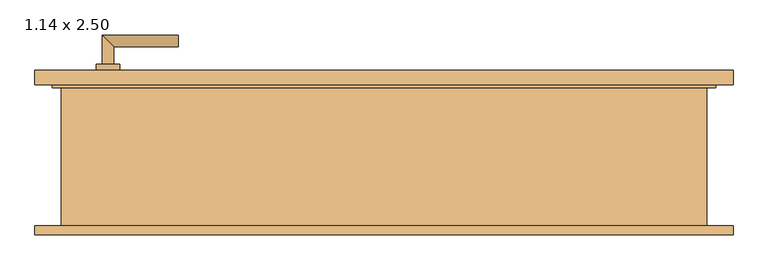
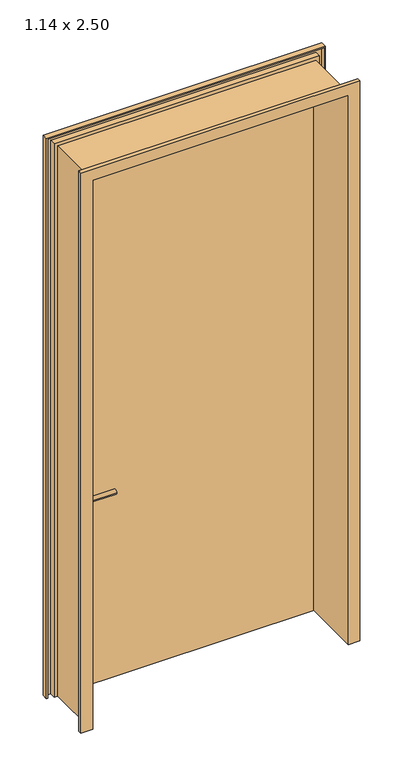
"""IFC4 building model written with IfcOpenShell, lengths in millimetres: door geometry, Drehflügel 1-flg - Stahlzarge : 1.14 x 2.50."""

from ifc_helpers import new_model, si_unit, point, frame, frame_2d, origin, place, context, project, spatial, polyline, circle_curve, ellipse_curve, trimmed, segment, composite_curve, outline, extrude, faceted_brep, source, transform, mapped, element, save
from ifc_brep_helpers import plane_surface, cylinder_surface, advanced_brep


def door_1_14_x_2_50_9918e422(model_context):
    return source(origin(), model_context, "Body", "SolidModel", [
        advanced_brep(
        [(-480.0, 109.4346141, 1000.0), (-460.0, 109.4346141, 1000.0), (-480.0, 39.4346141, 1000.0), (-460.0, 59.4346141, 1000.0), (-350.0, 39.4346141, 1000.0), (-350.0, 59.4346141, 1000.0)],
        [
            (0, 1, circle_curve(frame((-470.0, 109.4346141, 1000.0), z_axis=(0.0, 1.0, 0.0), x_axis=(1.0, 0.0, 0.0)), 10.0)),
            (1, 0, circle_curve(frame((-470.0, 109.4346141, 1000.0), z_axis=(0.0, 1.0, 0.0), x_axis=(1.0, 0.0, 0.0)), 10.0)),
            (0, 2),
            (2, 3, ellipse_curve(frame((-470.0, 49.4346141, 1000.0), z_axis=(-0.7071067811865385, 0.7071067811865565, 0.0), x_axis=(0.7071067811865563, 0.7071067811865386, 0.0)), 14.1421356, 10.0)),
            (3, 1),
            (3, 2, ellipse_curve(frame((-470.0, 49.4346141, 1000.0), z_axis=(-0.7071067811865385, 0.7071067811865565, 0.0), x_axis=(0.7071067811865563, 0.7071067811865386, 0.0)), 14.1421356, 10.0)),
            (4, 5, circle_curve(frame((-350.0, 49.4346141, 1000.0), z_axis=(1.0, 0.0, 0.0), x_axis=(0.0, 1.0, 0.0)), 10.0)),
            (5, 4, circle_curve(frame((-350.0, 49.4346141, 1000.0), z_axis=(1.0, 0.0, 0.0), x_axis=(0.0, 1.0, 0.0)), 10.0)),
            (2, 4),
            (5, 3),
        ],
        [
            plane_surface(frame((-470.0, 109.4346141, -287.7526403), z_axis=(0.0, 1.0, 0.0), x_axis=(0.0, 0.0, 1.0))),
            cylinder_surface(frame((-470.0, 109.4346141, 1000.0), z_axis=(0.0, 1.0, 0.0), x_axis=(1.0, 0.0, 0.0)), 10.0),
            plane_surface(frame((-350.0, 49.4346141, -287.7526403), z_axis=(1.0, 0.0, 0.0), x_axis=(0.0, 0.0, 1.0))),
            cylinder_surface(frame((-470.0, 49.4346141, 1000.0), z_axis=(-1.0, 0.0, 0.0), x_axis=(0.0, 1.0, 0.0)), 10.0),
        ],
        [
            (0, [[1, 2]]),
            (1, [[-1, 3, 4, 5]]),
            (1, [[-2, -5, 6, -3]]),
            (2, [[7, 8]]),
            (3, [[-4, 9, -8, 10]]),
            (3, [[-6, -10, -7, -9]]),
        ],
    ),
        advanced_brep(
        [(-460.0, 169.4346141, 1000.0), (-480.0, 169.4346141, 1000.0), (-460.0, 199.4346141, 1000.0), (-480.0, 219.4346141, 1000.0), (-350.0, 199.4346141, 1000.0), (-350.0, 219.4346141, 1000.0)],
        [
            (0, 1, circle_curve(frame((-470.0, 169.4346141, 1000.0), z_axis=(0.0, -1.0, 0.0), x_axis=(-1.0, 0.0, 0.0)), 10.0)),
            (1, 0, circle_curve(frame((-470.0, 169.4346141, 1000.0), z_axis=(0.0, -1.0, 0.0), x_axis=(-1.0, 0.0, 0.0)), 10.0)),
            (0, 2),
            (2, 3, ellipse_curve(frame((-470.0, 209.4346141, 1000.0), z_axis=(-0.7071067811865475, -0.7071067811865475, 0.0), x_axis=(0.7071067811865474, -0.7071067811865476, 0.0)), 14.1421356, 10.0)),
            (3, 1),
            (3, 2, ellipse_curve(frame((-470.0, 209.4346141, 1000.0), z_axis=(-0.7071067811865475, -0.7071067811865475, 0.0), x_axis=(0.7071067811865474, -0.7071067811865476, 0.0)), 14.1421356, 10.0)),
            (4, 5, circle_curve(frame((-350.0, 209.4346141, 1000.0), z_axis=(1.0, 0.0, 0.0), x_axis=(0.0, 1.0, 0.0)), 10.0)),
            (5, 4, circle_curve(frame((-350.0, 209.4346141, 1000.0), z_axis=(1.0, 0.0, 0.0), x_axis=(0.0, 1.0, 0.0)), 10.0)),
            (2, 4),
            (5, 3),
        ],
        [
            plane_surface(frame((-470.0, 169.4346141, -287.7526403), z_axis=(0.0, -1.0, 0.0), x_axis=(0.0, 0.0, 1.0))),
            cylinder_surface(frame((-470.0, 169.4346141, 1000.0), z_axis=(0.0, -1.0, 0.0), x_axis=(-1.0, 0.0, 0.0)), 10.0),
            plane_surface(frame((-350.0, 209.4346141, -287.7526403), z_axis=(1.0, 0.0, 0.0), x_axis=(0.0, 0.0, 1.0))),
            cylinder_surface(frame((-470.0, 209.4346141, 1000.0), z_axis=(-1.0, 0.0, 0.0), x_axis=(0.0, 1.0, 0.0)), 10.0),
        ],
        [
            (0, [[1, 2]]),
            (1, [[-1, 3, 4, 5]]),
            (1, [[-2, -5, 6, -3]]),
            (2, [[7, 8]]),
            (3, [[-4, 9, -8, 10]]),
            (3, [[-6, -10, -7, -9]]),
        ],
    ),
        extrude(outline(composite_curve([segment(trimmed(circle_curve(frame_2d((1000.0, -470.0)), 20.0), [point((1000.0, -490.0))], [point((1000.0, -450.0))], False, "CARTESIAN"), True, "CONTINUOUS"), segment(trimmed(circle_curve(frame_2d((1000.0, -470.0)), 20.0), [point((1000.0, -450.0))], [point((1000.0, -490.0))], False, "CARTESIAN"), True, "CONTINUOUS")], self_intersect=False)), frame((0.0, 99.4346141, 0.0), z_axis=(0.0, 1.0, 0.0), x_axis=(0.0, 0.0, 1.0)), (0.0, 0.0, 1.0), 10.0),
        extrude(outline(composite_curve([segment(trimmed(circle_curve(frame_2d((1000.0, -470.0)), 20.0), [point((1000.0, -490.0))], [point((1000.0, -450.0))], False, "CARTESIAN"), True, "CONTINUOUS"), segment(trimmed(circle_curve(frame_2d((1000.0, -470.0)), 20.0), [point((1000.0, -450.0))], [point((1000.0, -490.0))], False, "CARTESIAN"), True, "CONTINUOUS")], self_intersect=False)), frame((0.0, 159.4346141, 0.0), z_axis=(0.0, 1.0, 0.0), x_axis=(0.0, 0.0, 1.0)), (0.0, 0.0, 1.0), 10.0),
        extrude(outline(polyline([(560.0, 134.4346141), (-560.0, 134.4346141), (-560.0, 159.4346141), (560.0, 159.4346141), (560.0, 134.4346141)])), frame((0.0, 0.0, 100.0), z_axis=(0.0, 0.0, 1.0), x_axis=(1.0, 0.0, 0.0)), (0.0, 0.0, 1.0), 2490.0),
        faceted_brep([(594.4603207, -120.5653859, 100.0), (545.0, -120.5653859, 100.0), (545.0, 134.4346141, 100.0), (560.0, 134.4346141, 100.0), (560.0, 159.4346141, 100.0), (594.4603207, 159.4346141, 100.0), (594.4603207, 134.4346141, 100.0), (589.4603207, 134.4346141, 100.0), (589.4603207, 154.4346141, 100.0), (565.0, 154.4346141, 100.0), (565.0, 129.4346141, 100.0), (550.0, 129.4346141, 100.0), (550.0, -115.5653859, 100.0), (589.4603207, -115.5653859, 100.0), (589.4603207, -105.5653859, 100.0), (594.4603207, -105.5653859, 100.0), (594.4603207, -120.5653859, 2624.4603207), (-594.4603207, -120.5653859, 2624.4603207), (-594.4603207, -120.5653859, 100.0), (-545.0, -120.5653859, 100.0), (-545.0, -120.5653859, 2575.0), (545.0, -120.5653859, 2575.0), (545.0, 134.4346141, 2575.0), (-545.0, 134.4346141, 2575.0), (-545.0, 134.4346141, 100.0), (-560.0, 134.4346141, 100.0), (-560.0, 134.4346141, 2590.0), (560.0, 134.4346141, 2590.0), (560.0, 159.4346141, 2590.0), (-560.0, 159.4346141, 2590.0), (-560.0, 159.4346141, 100.0), (-594.4603207, 159.4346141, 100.0), (-594.4603207, 159.4346141, 2624.4603207), (594.4603207, 159.4346141, 2624.4603207), (594.4603207, 134.4346141, 2624.4603207), (-594.4603207, 134.4346141, 2624.4603207), (-594.4603207, 134.4346141, 100.0), (-589.4603207, 134.4346141, 100.0), (-589.4603207, 134.4346141, 2619.4603207), (589.4603207, 134.4346141, 2619.4603207), (589.4603207, 154.4346141, 2619.4603207), (-589.4603207, 154.4346141, 2619.4603207), (-589.4603207, 154.4346141, 100.0), (-565.0, 154.4346141, 100.0), (-565.0, 154.4346141, 2595.0), (565.0, 154.4346141, 2595.0), (565.0, 129.4346141, 2595.0), (-565.0, 129.4346141, 2595.0), (-565.0, 129.4346141, 100.0), (-550.0, 129.4346141, 100.0), (-550.0, 129.4346141, 2580.0), (550.0, 129.4346141, 2580.0), (550.0, -115.5653859, 2580.0), (-550.0, -115.5653859, 2580.0), (-550.0, -115.5653859, 100.0), (-589.4603207, -115.5653859, 100.0), (-589.4603207, -115.5653859, 2619.4603207), (589.4603207, -115.5653859, 2619.4603207), (589.4603207, -105.5653859, 2619.4603207), (-589.4603207, -105.5653859, 2619.4603207), (-589.4603207, -105.5653859, 100.0), (-594.4603207, -105.5653859, 100.0), (-594.4603207, -105.5653859, 2624.4603207), (594.4603207, -105.5653859, 2624.4603207)], [[[0, 1, 2, 3, 4, 5, 6, 7, 8, 9, 10, 11, 12, 13, 14, 15]], [[1, 0, 16, 17, 18, 19, 20, 21]], [[2, 1, 21, 22]], [[3, 2, 22, 23, 24, 25, 26, 27]], [[4, 3, 27, 28]], [[5, 4, 28, 29, 30, 31, 32, 33]], [[6, 5, 33, 34]], [[7, 6, 34, 35, 36, 37, 38, 39]], [[8, 7, 39, 40]], [[9, 8, 40, 41, 42, 43, 44, 45]], [[10, 9, 45, 46]], [[11, 10, 46, 47, 48, 49, 50, 51]], [[12, 11, 51, 52]], [[13, 12, 52, 53, 54, 55, 56, 57]], [[14, 13, 57, 58]], [[15, 14, 58, 59, 60, 61, 62, 63]], [[0, 15, 63, 16]], [[17, 62, 61, 18]], [[18, 61, 60, 55, 54, 49, 48, 43, 42, 37, 36, 31, 30, 25, 24, 19]], [[23, 20, 19, 24]], [[29, 26, 25, 30]], [[35, 32, 31, 36]], [[41, 38, 37, 42]], [[47, 44, 43, 48]], [[53, 50, 49, 54]], [[59, 56, 55, 60]], [[22, 21, 20, 23]], [[28, 27, 26, 29]], [[34, 33, 32, 35]], [[40, 39, 38, 41]], [[46, 45, 44, 47]], [[52, 51, 50, 53]], [[58, 57, 56, 59]], [[16, 63, 62, 17]]]),
    ])


if __name__ == "__main__":
    model = new_model("IFC4")
    model_context = context("Model", 3, world=origin())
    ifc_project = project(units=[si_unit("LENGTHUNIT", "METRE", prefix="MILLI")], contexts=[model_context])
    site = spatial("IfcSite", under=ifc_project)
    building = spatial("IfcBuilding", under=site)
    placement = place(None, origin())
    door_1_14_x_2_50_shape = door_1_14_x_2_50_9918e422(model_context)
    element("IfcDoor", 1, ObjectType="Drehflügel 1-flg - Stahlzarge : 1.14 x 2.50", at=placement, inside=building, context=model_context, shape_type="MappedRepresentation", body=[
        mapped(door_1_14_x_2_50_shape, transform((0.0, 0.0, 0.0), x_axis=(1.0, 0.0, 0.0), y_axis=(0.0, 1.0, 0.0), z_axis=(0.0, 0.0, 1.0))),
    ])
    save(model, "model.ifc")

# Revit data of these elements
# Type "Drehflügel 1-flg - Stahlzarge : 1.14 x 2.50"
#   Type Mark = "28"
#   Operation = "SingleSwingRight"
#   Keynote = "16.03"
#   Analytic Construction = "Metall"
#   Thermal Resistance (R) = 0.270117 (m²·K)/W
#   Heat Transfer Coefficient (U) = 3.7021 W/(m²·K)
#   Rough Width = 1.140 m
#   Rough Height [instance default] = 2.600 m
#   Höhe Türgriff [instance default] = 0.900 m
#   Height = 2.500 m
#   Fußbodenaufbau [instance default] = 0.100 m
#   Width = 1.140 m
#   Sichtbarkeit Sturzlinien [instance default] = yes
#   Türgriff auswählen [instance default] = element 221079
#   Türgriff [instance default] = none
#   Türflügel [instance default] = none
#   Rahmen/Pfosten [instance default] = Metall - Lackiert - Grau
#   Visual Light Transmittance = 0
#   Solar Heat Gain Coefficient = 0
#   Function = (empty or 0)
#   Wall Closure = (empty or 0)
# Element 1 (IfcDoor, "Drehflügel 1-flg - Stahlzarge : 1.14 x 2.50")
#   Materials on its faces: "Metall - Lackiert - Grau", "Metall - Chrom", "Holz - Birke"
# Materials
#   "Metall - Lackiert - Grau": class "Farbe 1", colour RGB 98 98 98, transparency 0, Cost = 0
#   "Metall - Chrom": class "Metall", colour RGB 247 247 247, transparency 0, Cost = 0
#   "Holz - Birke": class "Holz", colour RGB 213 164 103, transparency 0, Cost = 0
